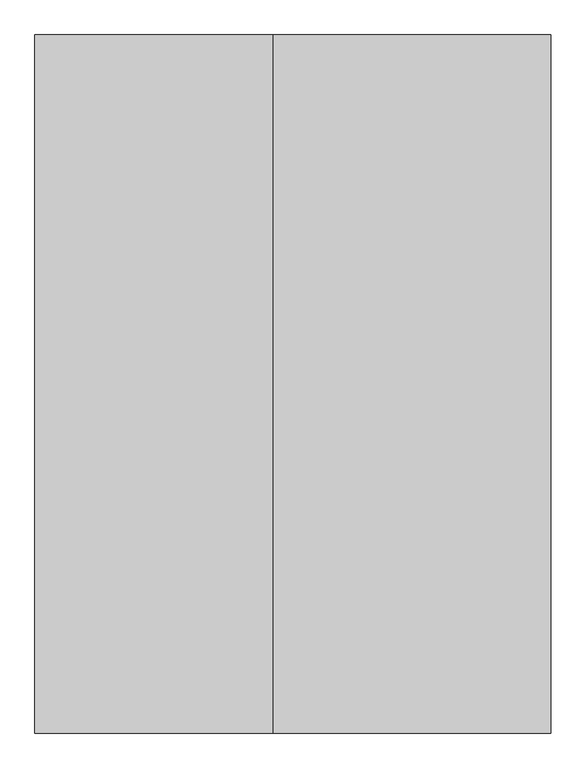
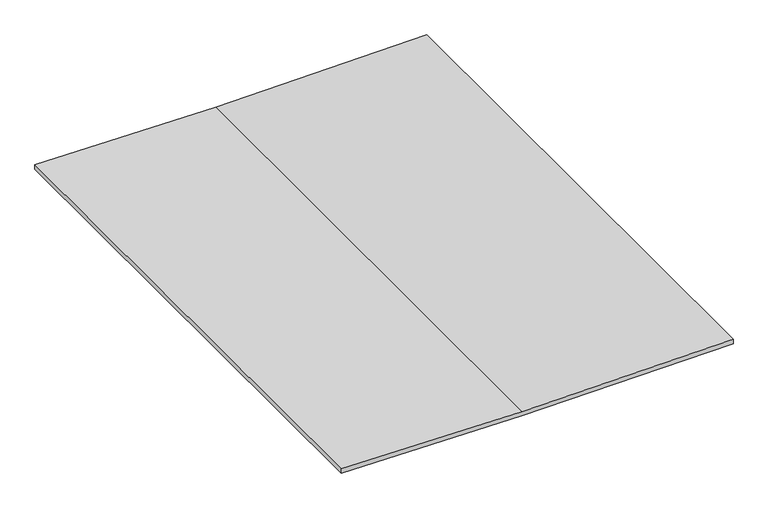
"""IFC4 building model written with IfcOpenShell, lengths in millimetres: proxy geometry, COVER BOARD 1:COVER BOARD 15441:299752 : COVER BOARD 1:COVER BOARD 15441:299752."""

from ifc_helpers import new_model, si_unit, frame, origin, place, context, project, spatial, polyline, outline, extrude, source, transform, mapped, element, save


def generic_models_86eb2abd(model_context):
    return source(origin(), model_context, "Body", "SweptSolid", [
        extrude(outline(polyline([(40237.9000089, 3686.9275669), (40228.1021556, 2890.4461596), (40237.9000089, 2209.6354065), (40220.5682898, 2209.6354065), (40210.7704365, 2890.4461596), (40220.5682898, 3686.9275669), (40237.9000089, 3686.9275669)])), frame((0.0, -774.3081162, 0.0), z_axis=(0.0, 1.0, 0.0), x_axis=(0.0, 0.0, 1.0)), (0.0, 0.0, 1.0), 2000.0),
    ])


if __name__ == "__main__":
    model = new_model("IFC4")
    model_context = context("Model", 3, world=origin())
    ifc_project = project(units=[si_unit("LENGTHUNIT", "METRE", prefix="MILLI")], contexts=[model_context])
    site = spatial("IfcSite", under=ifc_project)
    building = spatial("IfcBuilding", under=site)
    placement = place(None, origin())
    generic_models_shape = generic_models_86eb2abd(model_context)
    element("IfcBuildingElementProxy", 1, Name="COVER BOARD 1:COVER BOARD 15441:299752 : COVER BOARD 1:COVER BOARD 15441:299752", ObjectType="COVER BOARD 1:COVER BOARD 15441:299752 : COVER BOARD 1:COVER BOARD 15441:299752", at=placement, inside=building, context=model_context, shape_type="MappedRepresentation", body=[
        mapped(generic_models_shape, transform((0.0, 0.0, 0.0), x_axis=(1.0, 0.0, 0.0), y_axis=(0.0, 1.0, 0.0), z_axis=(0.0, 0.0, 1.0))),
    ])
    save(model, "model.ifc")

# Revit data of these elements
# Type "COVER BOARD 1:COVER BOARD 15441:299752 : COVER BOARD 1:COVER BOARD 15441:299752"
#   NameOverride = "COVER BOARD 1:COVER BOARD 15441:299752"
#   ObjectTypeOverride = "COVER BOARD 1:COVER BOARD 15441"
#   Reference = "COVER BOARD 15441"
#   Category = "Generic Models"
#   Tag = "299752"
# Element 1 (IfcBuildingElementProxy, "COVER BOARD 1:COVER BOARD 15441:299752 : COVER BOARD 1:COVER BOARD 15441:299752")
#   Materials on its faces: "CDX PLYWOOD - SEE STRUCTURAL DWGS"
# Materials
#   "CDX PLYWOOD - SEE STRUCTURAL DWGS": class "Unassigned", colour RGB 202 163 108, transparency 0, Cost = 0
